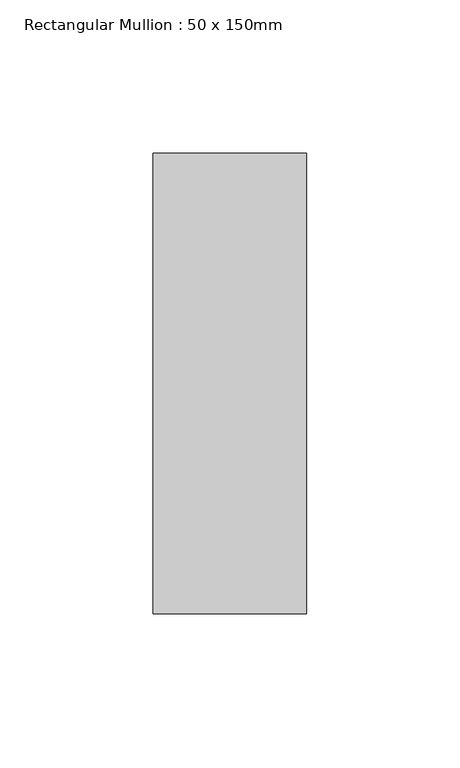
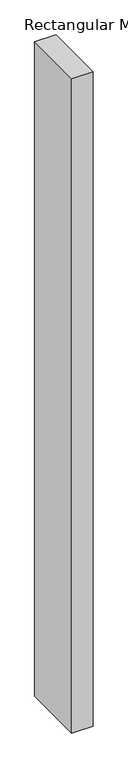
"""IFC4 building model written with IfcOpenShell, lengths in millimetres: member geometry, Rectangular Mullion : 50 x 150mm."""

from ifc_helpers import new_model, si_unit, frame, origin, place, context, project, spatial, polyline, outline, extrude, source, transform, mapped, element, save


def rectangular_mullion_50_x_150mm_d5096e64(model_context):
    return source(origin(), model_context, "Body", "SweptSolid", [
        extrude(outline(polyline([(25.0, 75.0), (25.0, -75.0), (-25.0, -75.0), (-25.0, 75.0), (25.0, 75.0)])), frame((0.0, 0.0, -1620.0), z_axis=(0.0, 0.0, 1.0), x_axis=(1.0, 0.0, 0.0)), (0.0, 0.0, 1.0), 1620.0),
    ])


if __name__ == "__main__":
    model = new_model("IFC4")
    model_context = context("Model", 3, world=origin())
    ifc_project = project(units=[si_unit("LENGTHUNIT", "METRE", prefix="MILLI")], contexts=[model_context])
    site = spatial("IfcSite", under=ifc_project)
    building = spatial("IfcBuilding", under=site)
    placement = place(None, origin())
    rectangular_mullion_50_x_150mm_shape = rectangular_mullion_50_x_150mm_d5096e64(model_context)
    element("IfcMember", 1, ObjectType="Rectangular Mullion : 50 x 150mm", at=placement, inside=building, context=model_context, shape_type="MappedRepresentation", body=[
        mapped(rectangular_mullion_50_x_150mm_shape, transform((0.0, 0.0, 0.0), x_axis=(1.0, 0.0, 0.0), y_axis=(0.0, 1.0, 0.0), z_axis=(0.0, 0.0, 1.0))),
    ])
    save(model, "model.ifc")

# Revit data of these elements
# Type "Rectangular Mullion : 50 x 150mm"
#   built-in parameter 1007304 = 0.492126 (stored number, unit not read)
#   built-in parameter 1007301 = 0.082021 (stored number, unit not read)
#   built-in parameter 1007300 = 0.082021 (stored number, unit not read)
# Element 1 (IfcMember, "Rectangular Mullion : 50 x 150mm")
#   Materials on its faces: "Metal - Aluminium"
# Materials
#   "Metal - Aluminium": class "Metal", colour RGB 247 247 247, transparency 0
